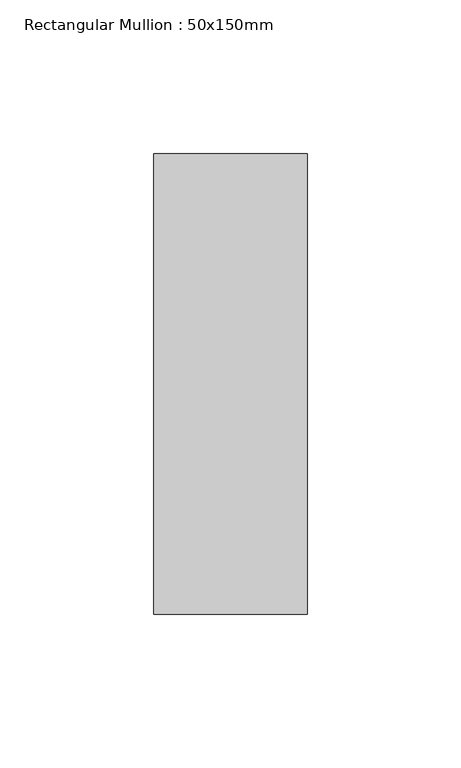
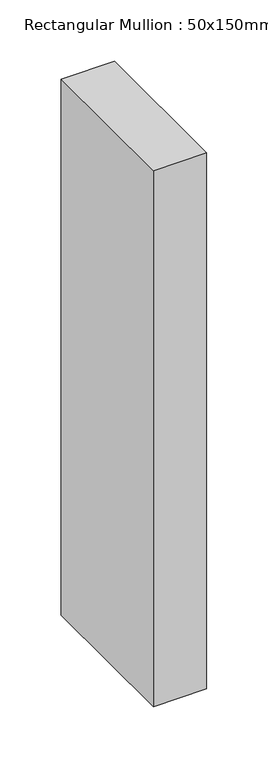
"""IFC4 building model written with IfcOpenShell, lengths in millimetres: member geometry, Rectangular Mullion : 50x150mm."""

from ifc_helpers import new_model, si_unit, frame, origin, place, context, project, spatial, polyline, outline, extrude, source, transform, mapped, element, save


def rectangular_mullion_50x150mm_bfadc177(model_context):
    return source(origin(), model_context, "Body", "SweptSolid", [
        extrude(outline(polyline([(0.0, 75.0), (0.0, -75.0), (-50.0, -75.0), (-50.0, 75.0), (0.0, 75.0)])), frame((0.0, 0.0, -532.5), z_axis=(0.0, 0.0, 1.0), x_axis=(1.0, 0.0, 0.0)), (0.0, 0.0, 1.0), 532.5),
    ])


if __name__ == "__main__":
    model = new_model("IFC4")
    model_context = context("Model", 3, world=origin())
    ifc_project = project(units=[si_unit("LENGTHUNIT", "METRE", prefix="MILLI")], contexts=[model_context])
    site = spatial("IfcSite", under=ifc_project)
    building = spatial("IfcBuilding", under=site)
    placement = place(None, origin())
    rectangular_mullion_50x150mm_shape = rectangular_mullion_50x150mm_bfadc177(model_context)
    element("IfcMember", 1, ObjectType="Rectangular Mullion : 50x150mm", at=placement, inside=building, context=model_context, shape_type="MappedRepresentation", body=[
        mapped(rectangular_mullion_50x150mm_shape, transform((0.0, 0.0, 0.0), x_axis=(1.0, 0.0, 0.0), y_axis=(0.0, 1.0, 0.0), z_axis=(0.0, 0.0, 1.0))),
    ])
    save(model, "model.ifc")

# Revit data of these elements
# Type "Rectangular Mullion : 50x150mm"
#   Keynote = "H11"
#   built-in parameter 1007304 = 0.492126 (stored number, unit not read)
#   built-in parameter 1007301 = 0.082021 (stored number, unit not read)
#   built-in parameter 1007300 = 0.082021 (stored number, unit not read)
# Element 1 (IfcMember, "Rectangular Mullion : 50x150mm")
#   Materials on its faces: "Aluminium"
# Materials
#   "Aluminium": class "Metal", colour RGB 247 247 247, transparency 0, Description = "Aluminium 6061", Cost = 0
